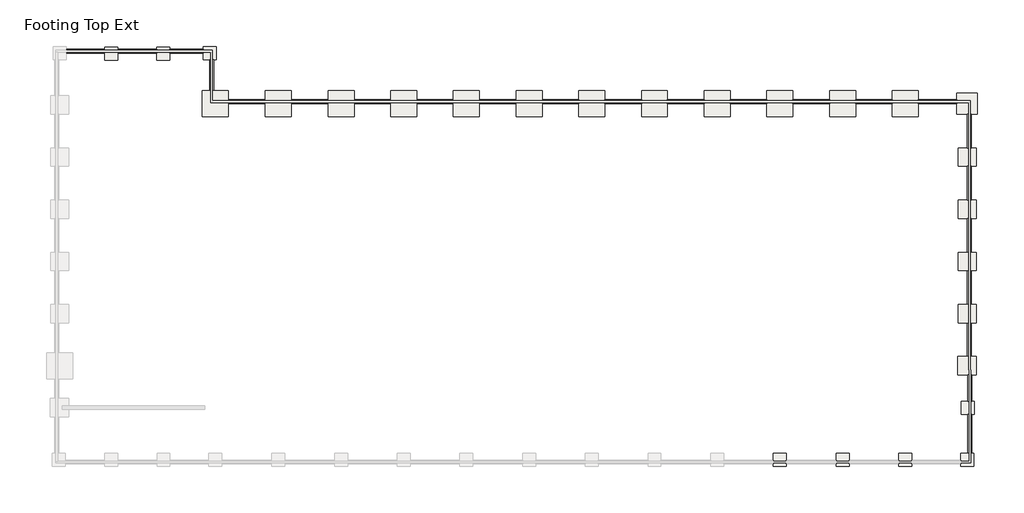
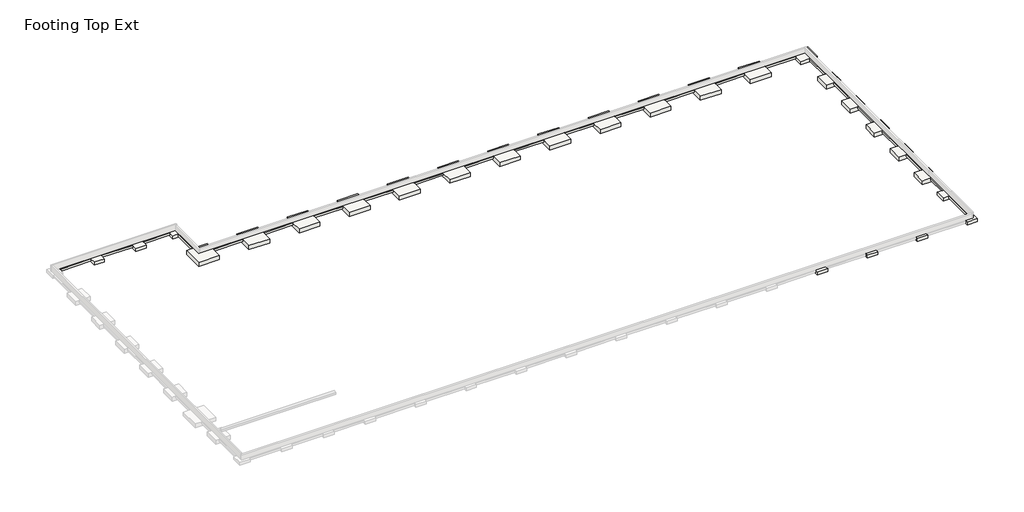
# One storey, part 2 of 2: 26 slabs, 5 footings.
"""IFC4 building model written with IfcOpenShell, lengths in millimetres."""

from ifc_helpers import new_model, si_unit, frame, origin, place, context, project, spatial, polyline, outline, extrude, faceted_brep, element, save

model = new_model("IFC4")

# Units and contexts
model_context = context("Model", 3, world=origin())
ifc_project = project(units=[si_unit("LENGTHUNIT", "METRE", prefix="MILLI")], contexts=[model_context])

# Site, building, storey
site = spatial("IfcSite", under=ifc_project)
building = spatial("IfcBuilding", under=site)
storey = spatial("IfcBuildingStorey", under=building, Name="Footing Top Ext", Elevation=-914.4)

# Footings
placement = place(None, origin())
element("IfcFooting", 1, ObjectType="Bearing Footing - 18\" x 12\"", at=placement, inside=storey, context=model_context, shape_type="SweptSolid", body=[
    extrude(outline(polyline([(305697.0398264, -530975.6413841), (305697.0398264, -530518.4413841), (310230.9398264, -530518.4413841), (310230.9398264, -530975.6413841), (305697.0398264, -530975.6413841)])), frame((0.0, 0.0, -1219.2), z_axis=(0.0, 0.0, 1.0), x_axis=(1.0, 0.0, 0.0)), (0.0, 0.0, 1.0), 304.8),
    extrude(outline(polyline([(317882.6898264, -530975.6413841), (317882.6898264, -530518.4413841), (321806.9898264, -530518.4413841), (321806.9898264, -530975.6413841), (317882.6898264, -530975.6413841)])), frame((0.0, 0.0, -1219.2), z_axis=(0.0, 0.0, 1.0), x_axis=(1.0, 0.0, 0.0)), (0.0, 0.0, 1.0), 304.8),
    extrude(outline(polyline([(316358.6898264, -530518.4413841), (316358.6898264, -530975.6413841), (311754.9398264, -530975.6413841), (311754.9398264, -530518.4413841), (316358.6898264, -530518.4413841)])), frame((0.0, 0.0, -1219.2), z_axis=(0.0, 0.0, 1.0), x_axis=(1.0, 0.0, 0.0)), (0.0, 0.0, 1.0), 304.8),
])
element("IfcFooting", 2, ObjectType="Bearing Footing - 18\" x 12\"", at=placement, inside=storey, context=model_context, shape_type="SweptSolid", body=[
    extrude(outline(polyline([(322537.2398264, -531712.2413841), (322994.4398264, -531712.2413841), (322994.4398264, -535382.5413841), (322537.2398264, -535382.5413841), (322537.2398264, -531712.2413841)])), frame((0.0, 0.0, -1219.2), z_axis=(0.0, 0.0, 1.0), x_axis=(1.0, 0.0, 0.0)), (0.0, 0.0, 1.0), 304.8),
])
element("IfcFooting", 3, ObjectType="Bearing Footing - 18\" x 12\"", at=placement, inside=storey, context=model_context, shape_type="SweptSolid", body=[
    extrude(outline(polyline([(410167.2397781, -536430.2913841), (410167.2397781, -536887.4913841), (405658.7398264, -536887.4913841), (405658.7398264, -536430.2913841), (410167.2397781, -536430.2913841)])), frame((0.0, 0.0, -1219.2), z_axis=(0.0, 0.0, 1.0), x_axis=(1.0, 0.0, 0.0)), (0.0, 0.0, 1.0), 304.8),
    extrude(outline(polyline([(402610.7398264, -536430.2913841), (402610.7398264, -536887.4913841), (398305.4398264, -536887.4913841), (398305.4398264, -536430.2913841), (402610.7398264, -536430.2913841)])), frame((0.0, 0.0, -1219.2), z_axis=(0.0, 0.0, 1.0), x_axis=(1.0, 0.0, 0.0)), (0.0, 0.0, 1.0), 304.8),
    extrude(outline(polyline([(395257.4398264, -536430.2913841), (395257.4398264, -536887.4913841), (390952.1398264, -536887.4913841), (390952.1398264, -536430.2913841), (395257.4398264, -536430.2913841)])), frame((0.0, 0.0, -1219.2), z_axis=(0.0, 0.0, 1.0), x_axis=(1.0, 0.0, 0.0)), (0.0, 0.0, 1.0), 304.8),
    extrude(outline(polyline([(387904.1398264, -536430.2913841), (387904.1398264, -536887.4913841), (383598.8398264, -536887.4913841), (383598.8398264, -536430.2913841), (387904.1398264, -536430.2913841)])), frame((0.0, 0.0, -1219.2), z_axis=(0.0, 0.0, 1.0), x_axis=(1.0, 0.0, 0.0)), (0.0, 0.0, 1.0), 304.8),
    extrude(outline(polyline([(380550.8398264, -536430.2913841), (380550.8398264, -536887.4913841), (376245.5398264, -536887.4913841), (376245.5398264, -536430.2913841), (380550.8398264, -536430.2913841)])), frame((0.0, 0.0, -1219.2), z_axis=(0.0, 0.0, 1.0), x_axis=(1.0, 0.0, 0.0)), (0.0, 0.0, 1.0), 304.8),
    extrude(outline(polyline([(373197.5398264, -536430.2913841), (373197.5398264, -536887.4913841), (368892.2398264, -536887.4913841), (368892.2398264, -536430.2913841), (373197.5398264, -536430.2913841)])), frame((0.0, 0.0, -1219.2), z_axis=(0.0, 0.0, 1.0), x_axis=(1.0, 0.0, 0.0)), (0.0, 0.0, 1.0), 304.8),
    extrude(outline(polyline([(365844.2398264, -536430.2913841), (365844.2398264, -536887.4913841), (361538.9398264, -536887.4913841), (361538.9398264, -536430.2913841), (365844.2398264, -536430.2913841)])), frame((0.0, 0.0, -1219.2), z_axis=(0.0, 0.0, 1.0), x_axis=(1.0, 0.0, 0.0)), (0.0, 0.0, 1.0), 304.8),
    extrude(outline(polyline([(358490.9398264, -536430.2913841), (358490.9398264, -536887.4913841), (354185.6398264, -536887.4913841), (354185.6398264, -536430.2913841), (358490.9398264, -536430.2913841)])), frame((0.0, 0.0, -1219.2), z_axis=(0.0, 0.0, 1.0), x_axis=(1.0, 0.0, 0.0)), (0.0, 0.0, 1.0), 304.8),
    extrude(outline(polyline([(351137.6398264, -536430.2913841), (351137.6398264, -536887.4913841), (346832.3398264, -536887.4913841), (346832.3398264, -536430.2913841), (351137.6398264, -536430.2913841)])), frame((0.0, 0.0, -1219.2), z_axis=(0.0, 0.0, 1.0), x_axis=(1.0, 0.0, 0.0)), (0.0, 0.0, 1.0), 304.8),
    extrude(outline(polyline([(343784.3398264, -536430.2913841), (343784.3398264, -536887.4913841), (339479.0398264, -536887.4913841), (339479.0398264, -536430.2913841), (343784.3398264, -536430.2913841)])), frame((0.0, 0.0, -1219.2), z_axis=(0.0, 0.0, 1.0), x_axis=(1.0, 0.0, 0.0)), (0.0, 0.0, 1.0), 304.8),
    extrude(outline(polyline([(336431.0398264, -536430.2913841), (336431.0398264, -536887.4913841), (332125.7398264, -536887.4913841), (332125.7398264, -536430.2913841), (336431.0398264, -536430.2913841)])), frame((0.0, 0.0, -1219.2), z_axis=(0.0, 0.0, 1.0), x_axis=(1.0, 0.0, 0.0)), (0.0, 0.0, 1.0), 304.8),
    extrude(outline(polyline([(329077.7398264, -536430.2913841), (329077.7398264, -536887.4913841), (324747.0398264, -536887.4913841), (324747.0398264, -536430.2913841), (329077.7398264, -536430.2913841)])), frame((0.0, 0.0, -1219.2), z_axis=(0.0, 0.0, 1.0), x_axis=(1.0, 0.0, 0.0)), (0.0, 0.0, 1.0), 304.8),
])
element("IfcFooting", 4, ObjectType="Bearing Footing - 18\" x 12\"", at=placement, inside=storey, context=model_context, shape_type="SweptSolid", body=[
    extrude(outline(polyline([(411894.4398264, -560496.7913841), (411437.2398264, -560496.7913841), (411437.2398264, -556502.6413841), (411894.4398264, -556502.6413841), (411894.4398264, -560496.7913841)])), frame((0.0, 0.0, -1219.2), z_axis=(0.0, 0.0, 1.0), x_axis=(1.0, 0.0, 0.0)), (0.0, 0.0, 1.0), 304.8),
    extrude(outline(polyline([(411437.2398264, -562630.3913841), (411894.4398264, -562630.3913841), (411894.4398264, -566599.1414082), (411437.2398264, -566599.1414082), (411437.2398264, -562630.3913841)])), frame((0.0, 0.0, -1219.2), z_axis=(0.0, 0.0, 1.0), x_axis=(1.0, 0.0, 0.0)), (0.0, 0.0, 1.0), 304.8),
    extrude(outline(polyline([(411894.4398264, -554369.0413841), (411437.2398264, -554369.0413841), (411437.2398264, -550374.8913841), (411894.4398264, -550374.8913841), (411894.4398264, -554369.0413841)])), frame((0.0, 0.0, -1219.2), z_axis=(0.0, 0.0, 1.0), x_axis=(1.0, 0.0, 0.0)), (0.0, 0.0, 1.0), 304.8),
    extrude(outline(polyline([(411894.4398264, -548241.2913841), (411437.2398264, -548241.2913841), (411437.2398264, -544247.1413841), (411894.4398264, -544247.1413841), (411894.4398264, -548241.2913841)])), frame((0.0, 0.0, -1219.2), z_axis=(0.0, 0.0, 1.0), x_axis=(1.0, 0.0, 0.0)), (0.0, 0.0, 1.0), 304.8),
    extrude(outline(polyline([(411894.4398264, -542113.5413841), (411437.2398264, -542113.5413841), (411437.2398264, -538119.3913358), (411894.4398264, -538119.3913358), (411894.4398264, -542113.5413841)])), frame((0.0, 0.0, -1219.2), z_axis=(0.0, 0.0, 1.0), x_axis=(1.0, 0.0, 0.0)), (0.0, 0.0, 1.0), 304.8),
])
element("IfcFooting", 5, ObjectType="Bearing Footing - 18\" x 12\"", at=placement, inside=storey, context=model_context, shape_type="SweptSolid", body=[
    extrude(outline(polyline([(411945.2398264, -577927.5413841), (411488.0398264, -577927.5413841), (411488.0398264, -573355.5413841), (411945.2398264, -573355.5413841), (411945.2398264, -577927.5413841)])), frame((0.0, 0.0, -1219.2), z_axis=(0.0, 0.0, 1.0), x_axis=(1.0, 0.0, 0.0)), (0.0, 0.0, 1.0), 304.8),
    extrude(outline(polyline([(411945.2398264, -571831.5413841), (411488.0398264, -571831.5413841), (411488.0398264, -568732.7414082), (411945.2398264, -568732.7414082), (411945.2398264, -571831.5413841)])), frame((0.0, 0.0, -1219.2), z_axis=(0.0, 0.0, 1.0), x_axis=(1.0, 0.0, 0.0)), (0.0, 0.0, 1.0), 304.8),
])

# Slabs
element("IfcSlab", 6, ObjectType="Footing-Rectangular : F10", at=placement, inside=storey, context=model_context, shape_type="Brep", body=[
    faceted_brep([(402610.7398264, -535382.5413358, -914.4), (402610.7398264, -536430.2913841, -914.4), (402610.7398264, -536887.4913841, -914.4), (402610.7398264, -538430.5413358, -914.4), (405658.7398264, -538430.5413358, -914.4), (405658.7398264, -536887.4913841, -914.4), (405658.7398264, -536430.2913841, -914.4), (405658.7398264, -535382.5413358, -914.4), (402610.7398264, -535382.5413358, -1524.0), (405658.7398264, -535382.5413358, -1524.0), (405658.7398264, -538430.5413358, -1524.0), (402610.7398264, -538430.5413358, -1524.0)], [[[0, 1, 2, 3, 4, 5, 6, 7]], [[8, 9, 10, 11]], [[3, 2, 1, 0, 8, 11]], [[4, 3, 11, 10]], [[7, 6, 5, 4, 10, 9]], [[0, 7, 9, 8]]]),
])
element("IfcSlab", 7, ObjectType="Footing-Rectangular : F10", at=placement, inside=storey, context=model_context, shape_type="Brep", body=[
    faceted_brep([(395257.4398264, -535382.5413358, -914.4), (395257.4398264, -536430.2913841, -914.4), (395257.4398264, -536887.4913841, -914.4), (395257.4398264, -538430.5413358, -914.4), (398305.4398264, -538430.5413358, -914.4), (398305.4398264, -536887.4913841, -914.4), (398305.4398264, -536430.2913841, -914.4), (398305.4398264, -535382.5413358, -914.4), (395257.4398264, -535382.5413358, -1524.0), (398305.4398264, -535382.5413358, -1524.0), (398305.4398264, -538430.5413358, -1524.0), (395257.4398264, -538430.5413358, -1524.0)], [[[0, 1, 2, 3, 4, 5, 6, 7]], [[8, 9, 10, 11]], [[3, 2, 1, 0, 8, 11]], [[4, 3, 11, 10]], [[7, 6, 5, 4, 10, 9]], [[0, 7, 9, 8]]]),
])
element("IfcSlab", 8, ObjectType="Footing-Rectangular : F10", at=placement, inside=storey, context=model_context, shape_type="Brep", body=[
    faceted_brep([(387904.1398264, -535382.5413358, -914.4), (387904.1398264, -536430.2913841, -914.4), (387904.1398264, -536887.4913841, -914.4), (387904.1398264, -538430.5413358, -914.4), (390952.1398264, -538430.5413358, -914.4), (390952.1398264, -536887.4913841, -914.4), (390952.1398264, -536430.2913841, -914.4), (390952.1398264, -535382.5413358, -914.4), (387904.1398264, -535382.5413358, -1524.0), (390952.1398264, -535382.5413358, -1524.0), (390952.1398264, -538430.5413358, -1524.0), (387904.1398264, -538430.5413358, -1524.0)], [[[0, 1, 2, 3, 4, 5, 6, 7]], [[8, 9, 10, 11]], [[3, 2, 1, 0, 8, 11]], [[4, 3, 11, 10]], [[7, 6, 5, 4, 10, 9]], [[0, 7, 9, 8]]]),
])
element("IfcSlab", 9, ObjectType="Footing-Rectangular : F10", at=placement, inside=storey, context=model_context, shape_type="Brep", body=[
    faceted_brep([(380550.8398264, -535382.5413358, -914.4), (380550.8398264, -536430.2913841, -914.4), (380550.8398264, -536887.4913841, -914.4), (380550.8398264, -538430.5413358, -914.4), (383598.8398264, -538430.5413358, -914.4), (383598.8398264, -536887.4913841, -914.4), (383598.8398264, -536430.2913841, -914.4), (383598.8398264, -535382.5413358, -914.4), (380550.8398264, -535382.5413358, -1524.0), (383598.8398264, -535382.5413358, -1524.0), (383598.8398264, -538430.5413358, -1524.0), (380550.8398264, -538430.5413358, -1524.0)], [[[0, 1, 2, 3, 4, 5, 6, 7]], [[8, 9, 10, 11]], [[3, 2, 1, 0, 8, 11]], [[4, 3, 11, 10]], [[7, 6, 5, 4, 10, 9]], [[0, 7, 9, 8]]]),
])
element("IfcSlab", 10, ObjectType="Footing-Rectangular : F10", at=placement, inside=storey, context=model_context, shape_type="Brep", body=[
    faceted_brep([(373197.5398264, -535382.5413358, -914.4), (373197.5398264, -536430.2913841, -914.4), (373197.5398264, -536887.4913841, -914.4), (373197.5398264, -538430.5413358, -914.4), (376245.5398264, -538430.5413358, -914.4), (376245.5398264, -536887.4913841, -914.4), (376245.5398264, -536430.2913841, -914.4), (376245.5398264, -535382.5413358, -914.4), (373197.5398264, -535382.5413358, -1524.0), (376245.5398264, -535382.5413358, -1524.0), (376245.5398264, -538430.5413358, -1524.0), (373197.5398264, -538430.5413358, -1524.0)], [[[0, 1, 2, 3, 4, 5, 6, 7]], [[8, 9, 10, 11]], [[3, 2, 1, 0, 8, 11]], [[4, 3, 11, 10]], [[7, 6, 5, 4, 10, 9]], [[0, 7, 9, 8]]]),
])
element("IfcSlab", 11, ObjectType="Footing-Rectangular : F10", at=placement, inside=storey, context=model_context, shape_type="Brep", body=[
    faceted_brep([(365844.2398264, -535382.5413358, -914.4), (365844.2398264, -536430.2913841, -914.4), (365844.2398264, -536887.4913841, -914.4), (365844.2398264, -538430.5413358, -914.4), (368892.2398264, -538430.5413358, -914.4), (368892.2398264, -536887.4913841, -914.4), (368892.2398264, -536430.2913841, -914.4), (368892.2398264, -535382.5413358, -914.4), (365844.2398264, -535382.5413358, -1524.0), (368892.2398264, -535382.5413358, -1524.0), (368892.2398264, -538430.5413358, -1524.0), (365844.2398264, -538430.5413358, -1524.0)], [[[0, 1, 2, 3, 4, 5, 6, 7]], [[8, 9, 10, 11]], [[3, 2, 1, 0, 8, 11]], [[4, 3, 11, 10]], [[7, 6, 5, 4, 10, 9]], [[0, 7, 9, 8]]]),
])
element("IfcSlab", 12, ObjectType="Footing-Rectangular : F10", at=placement, inside=storey, context=model_context, shape_type="Brep", body=[
    faceted_brep([(358490.9398264, -535382.5413358, -914.4), (358490.9398264, -536430.2913841, -914.4), (358490.9398264, -536887.4913841, -914.4), (358490.9398264, -538430.5413358, -914.4), (361538.9398264, -538430.5413358, -914.4), (361538.9398264, -536887.4913841, -914.4), (361538.9398264, -536430.2913841, -914.4), (361538.9398264, -535382.5413358, -914.4), (358490.9398264, -535382.5413358, -1524.0), (361538.9398264, -535382.5413358, -1524.0), (361538.9398264, -538430.5413358, -1524.0), (358490.9398264, -538430.5413358, -1524.0)], [[[0, 1, 2, 3, 4, 5, 6, 7]], [[8, 9, 10, 11]], [[3, 2, 1, 0, 8, 11]], [[4, 3, 11, 10]], [[7, 6, 5, 4, 10, 9]], [[0, 7, 9, 8]]]),
])
element("IfcSlab", 13, ObjectType="Footing-Rectangular : F10", at=placement, inside=storey, context=model_context, shape_type="Brep", body=[
    faceted_brep([(351137.6398264, -535382.5413358, -914.4), (351137.6398264, -536430.2913841, -914.4), (351137.6398264, -536887.4913841, -914.4), (351137.6398264, -538430.5413358, -914.4), (354185.6398264, -538430.5413358, -914.4), (354185.6398264, -536887.4913841, -914.4), (354185.6398264, -536430.2913841, -914.4), (354185.6398264, -535382.5413358, -914.4), (351137.6398264, -535382.5413358, -1524.0), (354185.6398264, -535382.5413358, -1524.0), (354185.6398264, -538430.5413358, -1524.0), (351137.6398264, -538430.5413358, -1524.0)], [[[0, 1, 2, 3, 4, 5, 6, 7]], [[8, 9, 10, 11]], [[3, 2, 1, 0, 8, 11]], [[4, 3, 11, 10]], [[7, 6, 5, 4, 10, 9]], [[0, 7, 9, 8]]]),
])
element("IfcSlab", 14, ObjectType="Footing-Rectangular : F10", at=placement, inside=storey, context=model_context, shape_type="Brep", body=[
    faceted_brep([(343784.3398264, -535382.5413358, -914.4), (343784.3398264, -536430.2913841, -914.4), (343784.3398264, -536887.4913841, -914.4), (343784.3398264, -538430.5413358, -914.4), (346832.3398264, -538430.5413358, -914.4), (346832.3398264, -536887.4913841, -914.4), (346832.3398264, -536430.2913841, -914.4), (346832.3398264, -535382.5413358, -914.4), (343784.3398264, -535382.5413358, -1524.0), (346832.3398264, -535382.5413358, -1524.0), (346832.3398264, -538430.5413358, -1524.0), (343784.3398264, -538430.5413358, -1524.0)], [[[0, 1, 2, 3, 4, 5, 6, 7]], [[8, 9, 10, 11]], [[3, 2, 1, 0, 8, 11]], [[4, 3, 11, 10]], [[7, 6, 5, 4, 10, 9]], [[0, 7, 9, 8]]]),
])
element("IfcSlab", 15, ObjectType="Footing-Rectangular : F10", at=placement, inside=storey, context=model_context, shape_type="Brep", body=[
    faceted_brep([(336431.0398264, -535382.5413358, -914.4), (336431.0398264, -536430.2913841, -914.4), (336431.0398264, -536887.4913841, -914.4), (336431.0398264, -538430.5413358, -914.4), (339479.0398264, -538430.5413358, -914.4), (339479.0398264, -536887.4913841, -914.4), (339479.0398264, -536430.2913841, -914.4), (339479.0398264, -535382.5413358, -914.4), (336431.0398264, -535382.5413358, -1524.0), (339479.0398264, -535382.5413358, -1524.0), (339479.0398264, -538430.5413358, -1524.0), (336431.0398264, -538430.5413358, -1524.0)], [[[0, 1, 2, 3, 4, 5, 6, 7]], [[8, 9, 10, 11]], [[3, 2, 1, 0, 8, 11]], [[4, 3, 11, 10]], [[7, 6, 5, 4, 10, 9]], [[0, 7, 9, 8]]]),
])
element("IfcSlab", 16, ObjectType="Footing-Rectangular : F10", at=placement, inside=storey, context=model_context, shape_type="Brep", body=[
    faceted_brep([(329077.7398264, -535382.5413358, -914.4), (329077.7398264, -536430.2913841, -914.4), (329077.7398264, -536887.4913841, -914.4), (329077.7398264, -538430.5413358, -914.4), (332125.7398264, -538430.5413358, -914.4), (332125.7398264, -536887.4913841, -914.4), (332125.7398264, -536430.2913841, -914.4), (332125.7398264, -535382.5413358, -914.4), (329077.7398264, -535382.5413358, -1524.0), (332125.7398264, -535382.5413358, -1524.0), (332125.7398264, -538430.5413358, -1524.0), (329077.7398264, -538430.5413358, -1524.0)], [[[0, 1, 2, 3, 4, 5, 6, 7]], [[8, 9, 10, 11]], [[3, 2, 1, 0, 8, 11]], [[4, 3, 11, 10]], [[7, 6, 5, 4, 10, 9]], [[0, 7, 9, 8]]]),
])
element("IfcSlab", 17, ObjectType="Footing-Rectangular : F10", at=placement, inside=storey, context=model_context, shape_type="Brep", body=[
    faceted_brep([(321699.0398264, -535382.5413841, -914.4), (321699.0398264, -538430.5413841, -914.4), (324747.0398264, -538430.5413841, -914.4), (324747.0398264, -536887.4913841, -914.4), (324747.0398264, -536430.2913841, -914.4), (324747.0398264, -535382.5413841, -914.4), (322994.4398264, -535382.5413841, -914.4), (322537.2398264, -535382.5413841, -914.4), (321699.0398264, -535382.5413841, -1524.0), (324747.0398264, -535382.5413841, -1524.0), (324747.0398264, -538430.5413841, -1524.0), (321699.0398264, -538430.5413841, -1524.0)], [[[0, 1, 2, 3, 4, 5, 6, 7]], [[8, 9, 10, 11]], [[1, 0, 8, 11]], [[2, 1, 11, 10]], [[5, 4, 3, 2, 10, 9]], [[0, 7, 6, 5, 9, 8]]]),
])
element("IfcSlab", 18, ObjectType="Footing-Rectangular : F5", at=placement, inside=storey, context=model_context, shape_type="Brep", body=[
    faceted_brep([(317882.6898264, -530245.3913841, -914.4), (316358.6898264, -530245.3913841, -914.4), (316358.6898264, -530518.4413841, -914.4), (316358.6898264, -530975.6413841, -914.4), (316358.6898264, -531769.3913841, -914.4), (317882.6898264, -531769.3913841, -914.4), (317882.6898264, -530975.6413841, -914.4), (317882.6898264, -530518.4413841, -914.4), (317882.6898264, -530245.3913841, -1371.6), (317882.6898264, -531769.3913841, -1371.6), (316358.6898264, -531769.3913841, -1371.6), (316358.6898264, -530245.3913841, -1371.6)], [[[0, 1, 2, 3, 4, 5, 6, 7]], [[8, 9, 10, 11]], [[1, 0, 8, 11]], [[4, 3, 2, 1, 11, 10]], [[5, 4, 10, 9]], [[0, 7, 6, 5, 9, 8]]]),
])
element("IfcSlab", 19, ObjectType="Footing-Rectangular : F5", at=placement, inside=storey, context=model_context, shape_type="Brep", body=[
    faceted_brep([(311754.9398264, -530245.3913841, -914.4), (310230.9398264, -530245.3913841, -914.4), (310230.9398264, -530518.4413841, -914.4), (310230.9398264, -530975.6413841, -914.4), (310230.9398264, -531769.3913841, -914.4), (311754.9398264, -531769.3913841, -914.4), (311754.9398264, -530975.6413841, -914.4), (311754.9398264, -530518.4413841, -914.4), (311754.9398264, -530245.3913841, -1371.6), (311754.9398264, -531769.3913841, -1371.6), (310230.9398264, -531769.3913841, -1371.6), (310230.9398264, -530245.3913841, -1371.6)], [[[0, 1, 2, 3, 4, 5, 6, 7]], [[8, 9, 10, 11]], [[1, 0, 8, 11]], [[4, 3, 2, 1, 11, 10]], [[5, 4, 10, 9]], [[0, 7, 6, 5, 9, 8]]]),
])
element("IfcSlab", 20, ObjectType="Footing-Rectangular : F5", at=placement, inside=storey, context=model_context, shape_type="Brep", body=[
    faceted_brep([(323330.9898264, -530188.2413841, -914.4), (321806.9898264, -530188.2413841, -914.4), (321806.9898264, -530518.4413841, -914.4), (321806.9898264, -530975.6413841, -914.4), (321806.9898264, -531712.2413841, -914.4), (322537.2398264, -531712.2413841, -914.4), (322994.4398264, -531712.2413841, -914.4), (323330.9898264, -531712.2413841, -914.4), (323330.9898264, -530188.2413841, -1371.6), (323330.9898264, -531712.2413841, -1371.6), (321806.9898264, -531712.2413841, -1371.6), (321806.9898264, -530188.2413841, -1371.6)], [[[0, 1, 2, 3, 4, 5, 6, 7]], [[8, 9, 10, 11]], [[1, 0, 8, 11]], [[4, 3, 2, 1, 11, 10]], [[7, 6, 5, 4, 10, 9]], [[0, 7, 9, 8]]]),
])
element("IfcSlab", 21, ObjectType="Footing-Rectangular : F5", at=placement, inside=storey, context=model_context, shape_type="Brep", body=[
    faceted_brep([(390190.1398264, -577978.3413841, -914.4), (388666.1398264, -577978.3413841, -914.4), (388666.1398264, -578759.3913841, -914.4), (388666.1398264, -579216.5913841, -914.4), (388666.1398264, -579502.3413841, -914.4), (390190.1398264, -579502.3413841, -914.4), (390190.1398264, -579216.5913841, -914.4), (390190.1398264, -578759.3913841, -914.4), (390190.1398264, -577978.3413841, -1371.6), (390190.1398264, -579502.3413841, -1371.6), (388666.1398264, -579502.3413841, -1371.6), (388666.1398264, -577978.3413841, -1371.6)], [[[0, 1, 2, 3, 4, 5, 6, 7]], [[8, 9, 10, 11]], [[1, 0, 8, 11]], [[4, 3, 2, 1, 11, 10]], [[5, 4, 10, 9]], [[0, 7, 6, 5, 9, 8]]]),
])
element("IfcSlab", 22, ObjectType="Footing-Rectangular : F5", at=placement, inside=storey, context=model_context, shape_type="Brep", body=[
    faceted_brep([(397543.4398264, -577971.9913841, -914.4), (396019.4398264, -577971.9913841, -914.4), (396019.4398264, -578759.3913841, -914.4), (396019.4398264, -579216.5913841, -914.4), (396019.4398264, -579495.9913841, -914.4), (397543.4398264, -579495.9913841, -914.4), (397543.4398264, -579216.5913841, -914.4), (397543.4398264, -578759.3913841, -914.4), (397543.4398264, -577971.9913841, -1371.6), (397543.4398264, -579495.9913841, -1371.6), (396019.4398264, -579495.9913841, -1371.6), (396019.4398264, -577971.9913841, -1371.6)], [[[0, 1, 2, 3, 4, 5, 6, 7]], [[8, 9, 10, 11]], [[1, 0, 8, 11]], [[4, 3, 2, 1, 11, 10]], [[5, 4, 10, 9]], [[0, 7, 6, 5, 9, 8]]]),
])
element("IfcSlab", 23, ObjectType="Footing-Rectangular : F5", at=placement, inside=storey, context=model_context, shape_type="Brep", body=[
    faceted_brep([(404896.7398264, -577971.9913841, -914.4), (403372.7398264, -577971.9913841, -914.4), (403372.7398264, -578759.3913841, -914.4), (403372.7398264, -579216.5913841, -914.4), (403372.7398264, -579495.9913841, -914.4), (404896.7398264, -579495.9913841, -914.4), (404896.7398264, -579216.5913841, -914.4), (404896.7398264, -578759.3913841, -914.4), (404896.7398264, -577971.9913841, -1371.6), (404896.7398264, -579495.9913841, -1371.6), (403372.7398264, -579495.9913841, -1371.6), (403372.7398264, -577971.9913841, -1371.6)], [[[0, 1, 2, 3, 4, 5, 6, 7]], [[8, 9, 10, 11]], [[1, 0, 8, 11]], [[4, 3, 2, 1, 11, 10]], [[5, 4, 10, 9]], [[0, 7, 6, 5, 9, 8]]]),
])
element("IfcSlab", 24, ObjectType="Footing-Rectangular : F5", at=placement, inside=storey, context=model_context, shape_type="Brep", body=[
    faceted_brep([(412199.2398264, -577927.5413841, -914.4), (411945.2398264, -577927.5413841, -914.4), (411488.0398264, -577927.5413841, -914.4), (410675.2398264, -577927.5413841, -914.4), (410675.2398264, -578759.3913841, -914.4), (410675.2398264, -579216.5913841, -914.4), (410675.2398264, -579451.5413841, -914.4), (412199.2398264, -579451.5413841, -914.4), (412199.2398264, -577927.5413841, -1371.6), (412199.2398264, -579451.5413841, -1371.6), (410675.2398264, -579451.5413841, -1371.6), (410675.2398264, -577927.5413841, -1371.6)], [[[0, 1, 2, 3, 4, 5, 6, 7]], [[8, 9, 10, 11]], [[3, 2, 1, 0, 8, 11]], [[6, 5, 4, 3, 11, 10]], [[7, 6, 10, 9]], [[0, 7, 9, 8]]]),
])
element("IfcSlab", 25, ObjectType="Footing-Rectangular : F5", at=placement, inside=storey, context=model_context, shape_type="Brep", body=[
    faceted_brep([(412218.2898264, -571831.5413841, -914.4), (411945.2398264, -571831.5413841, -914.4), (411488.0398264, -571831.5413841, -914.4), (410694.2898264, -571831.5413841, -914.4), (410694.2898264, -573355.5413841, -914.4), (411488.0398264, -573355.5413841, -914.4), (411945.2398264, -573355.5413841, -914.4), (412218.2898264, -573355.5413841, -914.4), (412218.2898264, -571831.5413841, -1371.6), (412218.2898264, -573355.5413841, -1371.6), (410694.2898264, -573355.5413841, -1371.6), (410694.2898264, -571831.5413841, -1371.6)], [[[0, 1, 2, 3, 4, 5, 6, 7]], [[8, 9, 10, 11]], [[3, 2, 1, 0, 8, 11]], [[4, 3, 11, 10]], [[7, 6, 5, 4, 10, 9]], [[0, 7, 9, 8]]]),
])
element("IfcSlab", 26, ObjectType="Footing-Rectangular : F7", at=placement, inside=storey, context=model_context, shape_type="Brep", body=[
    faceted_brep([(410319.6398264, -566599.1414082, -914.4), (410319.6398264, -568732.7414082, -914.4), (411488.0398264, -568732.7414082, -914.4), (411945.2398264, -568732.7414082, -914.4), (412453.2398264, -568732.7414082, -914.4), (412453.2398264, -566599.1414082, -914.4), (411894.4398264, -566599.1414082, -914.4), (411437.2398264, -566599.1414082, -914.4), (410319.6398264, -566599.1414082, -1524.0), (412453.2398264, -566599.1414082, -1524.0), (412453.2398264, -568732.7414082, -1524.0), (410319.6398264, -568732.7414082, -1524.0)], [[[0, 1, 2, 3, 4, 5, 6, 7]], [[8, 9, 10, 11]], [[1, 0, 8, 11]], [[4, 3, 2, 1, 11, 10]], [[5, 4, 10, 9]], [[0, 7, 6, 5, 9, 8]]]),
])
element("IfcSlab", 27, ObjectType="Footing-Rectangular : F7", at=placement, inside=storey, context=model_context, shape_type="Brep", body=[
    faceted_brep([(412484.9898264, -560496.7913841, -914.4), (411894.4398264, -560496.7913841, -914.4), (411437.2398264, -560496.7913841, -914.4), (410351.3898264, -560496.7913841, -914.4), (410351.3898264, -562630.3913841, -914.4), (411437.2398264, -562630.3913841, -914.4), (411894.4398264, -562630.3913841, -914.4), (412484.9898264, -562630.3913841, -914.4), (412484.9898264, -560496.7913841, -1524.0), (412484.9898264, -562630.3913841, -1524.0), (410351.3898264, -562630.3913841, -1524.0), (410351.3898264, -560496.7913841, -1524.0)], [[[0, 1, 2, 3, 4, 5, 6, 7]], [[8, 9, 10, 11]], [[3, 2, 1, 0, 8, 11]], [[4, 3, 11, 10]], [[7, 6, 5, 4, 10, 9]], [[0, 7, 9, 8]]]),
])
element("IfcSlab", 28, ObjectType="Footing-Rectangular : F7", at=placement, inside=storey, context=model_context, shape_type="Brep", body=[
    faceted_brep([(412484.9898264, -554369.0413841, -914.4), (411894.4398264, -554369.0413841, -914.4), (411437.2398264, -554369.0413841, -914.4), (410351.3898264, -554369.0413841, -914.4), (410351.3898264, -556502.6413841, -914.4), (411437.2398264, -556502.6413841, -914.4), (411894.4398264, -556502.6413841, -914.4), (412484.9898264, -556502.6413841, -914.4), (412484.9898264, -554369.0413841, -1524.0), (412484.9898264, -556502.6413841, -1524.0), (410351.3898264, -556502.6413841, -1524.0), (410351.3898264, -554369.0413841, -1524.0)], [[[0, 1, 2, 3, 4, 5, 6, 7]], [[8, 9, 10, 11]], [[3, 2, 1, 0, 8, 11]], [[4, 3, 11, 10]], [[7, 6, 5, 4, 10, 9]], [[0, 7, 9, 8]]]),
])
element("IfcSlab", 29, ObjectType="Footing-Rectangular : F7", at=placement, inside=storey, context=model_context, shape_type="Brep", body=[
    faceted_brep([(412484.9898264, -548241.2913841, -914.4), (411894.4398264, -548241.2913841, -914.4), (411437.2398264, -548241.2913841, -914.4), (410351.3898264, -548241.2913841, -914.4), (410351.3898264, -550374.8913841, -914.4), (411437.2398264, -550374.8913841, -914.4), (411894.4398264, -550374.8913841, -914.4), (412484.9898264, -550374.8913841, -914.4), (412484.9898264, -548241.2913841, -1524.0), (412484.9898264, -550374.8913841, -1524.0), (410351.3898264, -550374.8913841, -1524.0), (410351.3898264, -548241.2913841, -1524.0)], [[[0, 1, 2, 3, 4, 5, 6, 7]], [[8, 9, 10, 11]], [[3, 2, 1, 0, 8, 11]], [[4, 3, 11, 10]], [[7, 6, 5, 4, 10, 9]], [[0, 7, 9, 8]]]),
])
element("IfcSlab", 30, ObjectType="Footing-Rectangular : F7", at=placement, inside=storey, context=model_context, shape_type="Brep", body=[
    faceted_brep([(412478.6398264, -542113.5413841, -914.4), (411894.4398264, -542113.5413841, -914.4), (411437.2398264, -542113.5413841, -914.4), (410345.0398264, -542113.5413841, -914.4), (410345.0398264, -544247.1413841, -914.4), (411437.2398264, -544247.1413841, -914.4), (411894.4398264, -544247.1413841, -914.4), (412478.6398264, -544247.1413841, -914.4), (412478.6398264, -542113.5413841, -1524.0), (412478.6398264, -544247.1413841, -1524.0), (410345.0398264, -544247.1413841, -1524.0), (410345.0398264, -542113.5413841, -1524.0)], [[[0, 1, 2, 3, 4, 5, 6, 7]], [[8, 9, 10, 11]], [[3, 2, 1, 0, 8, 11]], [[4, 3, 11, 10]], [[7, 6, 5, 4, 10, 9]], [[0, 7, 9, 8]]]),
])
element("IfcSlab", 31, ObjectType="Footing-Rectangular : F8", at=placement, inside=storey, context=model_context, shape_type="Brep", body=[
    faceted_brep([(410167.2397781, -535680.9913358, -914.4), (410167.2397781, -536430.2913841, -914.4), (410167.2397781, -536887.4913841, -914.4), (410167.2397781, -538119.3913358, -914.4), (411437.2398264, -538119.3913358, -914.4), (411894.4398264, -538119.3913358, -914.4), (412605.6397781, -538119.3913358, -914.4), (412605.6397781, -535680.9913358, -914.4), (410167.2397781, -535680.9913358, -1371.6), (412605.6397781, -535680.9913358, -1371.6), (412605.6397781, -538119.3913358, -1371.6), (410167.2397781, -538119.3913358, -1371.6)], [[[0, 1, 2, 3, 4, 5, 6, 7]], [[8, 9, 10, 11]], [[3, 2, 1, 0, 8, 11]], [[6, 5, 4, 3, 11, 10]], [[7, 6, 10, 9]], [[0, 7, 9, 8]]]),
])

save(model, "model.ifc")

# Revit data of these elements
# Type "Bearing Footing - 18\" x 12\""
#   Assembly Code = "A1010110"
# Type "Footing-Rectangular : F10"
#   Assembly Code = "A1010100"
#   Width = 10' - 0"
#   Length = 10' - 0"
#   Thickness = 2' - 0"
#   Structural Material [instance default] = Concrete, Cast-in-Place gray
# Type "Footing-Rectangular : F5"
#   Assembly Code = "A1010100"
#   Width = 5' - 0"
#   Length = 5' - 0"
#   Thickness = 1' - 6"
#   Structural Material [instance default] = Concrete, Cast-in-Place gray
# Type "Footing-Rectangular : F7"
#   Assembly Code = "A1010100"
#   Width = 7' - 0"
#   Length = 7' - 0"
#   Thickness = 2' - 0"
#   Structural Material [instance default] = Concrete, Cast-in-Place gray
# Type "Footing-Rectangular : F8"
#   Assembly Code = "A1010100"
#   Width = 8' - 0"
#   Length = 8' - 0"
#   Thickness = 1' - 6"
#   Structural Material [instance default] = Concrete, Cast-in-Place gray
# Elements 1, 2, 3, 4, 5 (IfcFooting, "Bearing Footing - 18\" x 12\"")
#   Phase Created = New Construction
#   Materials on its faces: "Concrete, Cast-in-Place gray"
# Elements 6, 7, 8, 9, 10, 11, 12, 13, 14, 15, 16, 17 (IfcSlab, "Footing-Rectangular : F10")
#   Comments = ""
#   Structural Material = Concrete, Cast-in-Place gray
#   Phase Created = New Construction
#   Materials on its faces: "Concrete, Cast-in-Place gray"
# Elements 18, 19, 20, 21, 22, 23, 24, 25 (IfcSlab, "Footing-Rectangular : F5")
#   Comments = ""
#   Structural Material = Concrete, Cast-in-Place gray
#   Phase Created = New Construction
#   Materials on its faces: "Concrete, Cast-in-Place gray"
# Elements 26, 27, 28, 29, 30 (IfcSlab, "Footing-Rectangular : F7")
#   Comments = ""
#   Structural Material = Concrete, Cast-in-Place gray
#   Phase Created = New Construction
#   Materials on its faces: "Concrete, Cast-in-Place gray"
# Element 31 (IfcSlab, "Footing-Rectangular : F8")
#   Comments = ""
#   Structural Material = Concrete, Cast-in-Place gray
#   Phase Created = New Construction
#   Materials on its faces: "Concrete, Cast-in-Place gray"
# Materials
#   "Concrete, Cast-in-Place gray": class "Concrete", colour RGB 192 192 192, transparency 0, Description = "Cast-in-place concrete", Cost = 0
